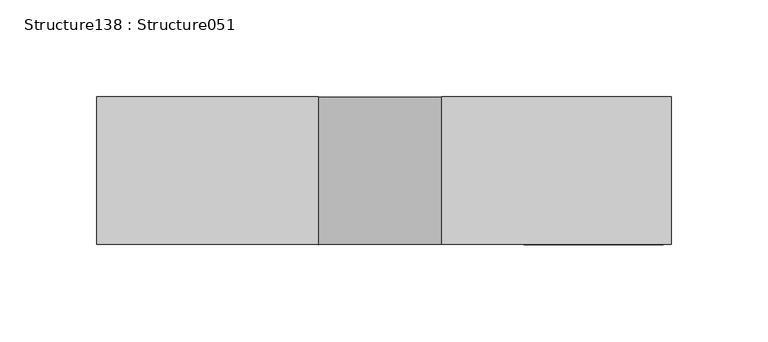
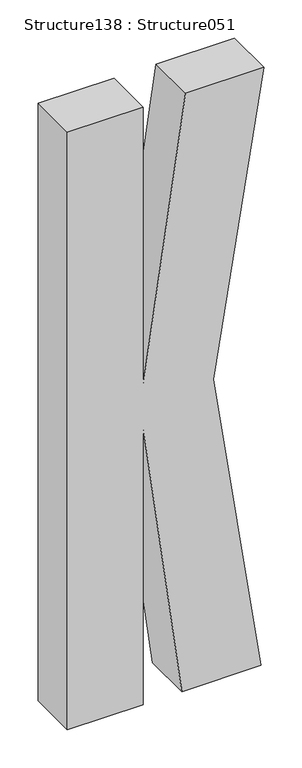
"""IFC4 building model written with IfcOpenShell, lengths in millimetres: proxy geometry, Structure138 : Structure051."""

import ifcopenshell
import ifcopenshell.guid

model = None  # the IFC model being written
_history = None  # IfcOwnerHistory: only IFC2X3 demands one
_inside = {}  # id of a spatial element -> (the spatial element, [elements in it])
_under = {}  # id of a project, library or spatial element -> (it, [spatial elements below it])
_declared = {}  # id of a project -> (the project, [libraries it declares])
_typed = {}  # id of a type object -> (the type object, [elements of that type])
_made_of = {}  # id of a material, layer set ... -> (it, [elements and type objects made of it])


def new_model(schema):
    """Start an empty IFC model of exactly this schema.

    Asked for "IFC4X3", IfcOpenShell would pick the latest addendum, in which some entities
    have other attributes; the version numbers below select the first issue.
    IFC2X3 requires an IfcOwnerHistory on every rooted entity: one is made here for all.
    """
    global model, _history
    if schema == "IFC4X3":
        model = ifcopenshell.file(schema_version=(4, 3, 0, 0))
    else:
        model = ifcopenshell.file(schema=schema)
    _inside.clear()
    _under.clear()
    _declared.clear()
    _typed.clear()
    _made_of.clear()
    _history = None
    if model.schema == "IFC2X3":
        org = make("IfcOrganization", Name="unknown")
        user = make(
            "IfcPersonAndOrganization",
            ThePerson=make("IfcPerson", FamilyName="unknown"),
            TheOrganization=org,
        )
        app = make(
            "IfcApplication",
            ApplicationDeveloper=org,
            Version="unknown",
            ApplicationFullName="unknown",
            ApplicationIdentifier="unknown",
        )
        _history = make(
            "IfcOwnerHistory",
            OwningUser=user,
            OwningApplication=app,
            ChangeAction="ADDED",
            CreationDate=0,
        )
    return model


def make(cls, **values):
    """One entity of the class cls with the attributes given. An attribute that is None is left unset."""
    return model.create_entity(
        cls, **{name: value for name, value in values.items() if value is not None}
    )


def rooted(cls, **values):
    """An entity with a GlobalId (a new one), such as an element, a storey or a relation."""
    return make(cls, GlobalId=ifcopenshell.guid.new(), OwnerHistory=_history, **values)


def si_unit(unit_type, name, prefix=None):
    """IfcSIUnit, for example si_unit("LENGTHUNIT", "METRE", prefix="MILLI")."""
    return make("IfcSIUnit", UnitType=unit_type, Prefix=prefix, Name=name)


def assignment(units):
    """IfcUnitAssignment: the units of a project."""
    return None if units is None else make("IfcUnitAssignment", Units=units)


def point(xyz):
    """IfcCartesianPoint."""
    return None if xyz is None else make("IfcCartesianPoint", Coordinates=xyz)


def direction(xyz):
    """IfcDirection."""
    return None if xyz is None else make("IfcDirection", DirectionRatios=xyz)


def frame(location, z_axis=None, x_axis=None):
    """IfcAxis2Placement3D, a coordinate frame: its origin and axes. An axis left out is left unset."""
    return make(
        "IfcAxis2Placement3D",
        Location=point(location),
        Axis=direction(z_axis),
        RefDirection=direction(x_axis),
    )


def origin():
    """The frame at (0, 0, 0) with its axes left unset."""
    return frame((0.0, 0.0, 0.0))


def place(relative_to, where):
    """IfcLocalPlacement: puts the frame where relative to a parent placement (None: the world)."""
    return make(
        "IfcLocalPlacement", PlacementRelTo=relative_to, RelativePlacement=where
    )


def context(
    kind, dimensions, precision=None, world=None, true_north=None, identifier=None
):
    """IfcGeometricRepresentationContext, for example the 3D "Model" context."""
    return make(
        "IfcGeometricRepresentationContext",
        ContextIdentifier=identifier,
        ContextType=kind,
        CoordinateSpaceDimension=dimensions,
        Precision=precision,
        WorldCoordinateSystem=world,
        TrueNorth=true_north,
    )


def project(units=None, contexts=None):
    """IfcProject with its units and contexts."""
    return rooted(
        "IfcProject",
        Name="project",
        RepresentationContexts=contexts,
        UnitsInContext=assignment(units),
    )


def spatial(cls, under=None, at=None, **own):
    """A site, building, storey or space (cls), placed at a placement, below another one or the project."""
    s = rooted(cls, ObjectPlacement=at, **own)
    if under is not None:
        _under.setdefault(under.id(), (under, []))[1].append(s)
    return s


def polyline(points):
    """IfcPolyline through the points."""
    return make("IfcPolyline", Points=[point(p) for p in points])


def outline(outer, holes=None, kind="AREA"):
    """IfcArbitraryClosedProfileDef: a profile drawn as a closed curve; with holes, ...WithVoids."""
    if holes is None:
        return make("IfcArbitraryClosedProfileDef", ProfileType=kind, OuterCurve=outer)
    return make(
        "IfcArbitraryProfileDefWithVoids",
        ProfileType=kind,
        OuterCurve=outer,
        InnerCurves=holes,
    )


def extrude(swept, where, along, depth):
    """IfcExtrudedAreaSolid: the profile swept, set in the frame where, extruded along a direction by depth."""
    return make(
        "IfcExtrudedAreaSolid",
        SweptArea=swept,
        Position=where,
        ExtrudedDirection=direction(along),
        Depth=depth,
    )


def shape(context_of_items, identifier, shape_type, items):
    """IfcShapeRepresentation: the items that make up one representation, for example the "Body"."""
    return make(
        "IfcShapeRepresentation",
        ContextOfItems=context_of_items,
        RepresentationIdentifier=identifier,
        RepresentationType=shape_type,
        Items=items,
    )


def source(mapping_origin, context_of_items, identifier, shape_type, items):
    """IfcRepresentationMap: a shape defined once, which mapped items show again and again."""
    return make(
        "IfcRepresentationMap",
        MappingOrigin=mapping_origin,
        MappedRepresentation=shape(context_of_items, identifier, shape_type, items),
    )


def transform(
    local_origin,
    x_axis=None,
    y_axis=None,
    z_axis=None,
    scale=None,
    scale2=None,
    scale3=None,
    uniform=True,
):
    """IfcCartesianTransformationOperator3D, or its non-uniform kind. x_axis, y_axis, z_axis: its Axis1, 2, 3."""
    if uniform:
        return make(
            "IfcCartesianTransformationOperator3D",
            Axis1=direction(x_axis),
            Axis2=direction(y_axis),
            LocalOrigin=point(local_origin),
            Scale=scale,
            Axis3=direction(z_axis),
        )
    return make(
        "IfcCartesianTransformationOperator3DnonUniform",
        Axis1=direction(x_axis),
        Axis2=direction(y_axis),
        LocalOrigin=point(local_origin),
        Scale=scale,
        Axis3=direction(z_axis),
        Scale2=scale2,
        Scale3=scale3,
    )


def mapped(mapping_source, mapping_target):
    """IfcMappedItem: shows the shape of a source again, moved by a transform."""
    return make(
        "IfcMappedItem", MappingSource=mapping_source, MappingTarget=mapping_target
    )


def made_of(thing, what):
    """Note that an element or type object is made of a material, layer set ...; save() writes the relation."""
    if what is not None:
        _made_of.setdefault(what.id(), (what, []))[1].append(thing)
    return thing


def element(
    cls,
    number,
    at=None,
    inside=None,
    cuts=None,
    type_object=None,
    material=None,
    context=None,
    identifier="Body",
    shape_type=None,
    held_by="IfcProductDefinitionShape",
    body=None,
    shapes=None,
    **own,
):
    """One element of the class cls, such as IfcWall. Its Tag is "e" and its number.

    at: its placement. inside: the storey or other place that contains it. cuts: it is an
    opening in that element (IfcRelVoidsElement). A single representation is given by context,
    identifier, shape_type and body (its items); several are given by shapes. held_by: the class
    of the entity that holds the representations. save() writes the other relations.
    """
    e = rooted(cls, Tag="e%d" % number, ObjectPlacement=at, **own)
    if body is not None:
        shapes = [shape(context, identifier, shape_type, body)]
    if shapes is not None:
        e.Representation = make(held_by, Representations=shapes)
    if inside is not None:
        _inside.setdefault(inside.id(), (inside, []))[1].append(e)
    if cuts is not None:
        rooted(
            "IfcRelVoidsElement", RelatingBuildingElement=cuts, RelatedOpeningElement=e
        )
    if type_object is not None:
        _typed.setdefault(type_object.id(), (type_object, []))[1].append(e)
    return made_of(e, material)


def aggregate(whole, parts):
    """IfcRelAggregates: a whole, such as a stair, and the parts it consists of."""
    return rooted("IfcRelAggregates", RelatingObject=whole, RelatedObjects=parts)


def save(model, path):
    """Write the relations noted so far, then the file.

    IfcRelAggregates (storeys below a building ...), IfcRelContainedInSpatialStructure (elements
    in a storey), IfcRelDefinesByType, IfcRelAssociatesMaterial and IfcRelDeclares: one each for
    every whole, place, type object, material and project.
    """
    for whole, parts in _under.values():
        aggregate(whole, parts)
    for where, things in _inside.values():
        rooted(
            "IfcRelContainedInSpatialStructure",
            RelatedElements=things,
            RelatingStructure=where,
        )
    for kind, things in _typed.values():
        rooted("IfcRelDefinesByType", RelatedObjects=things, RelatingType=kind)
    for what, things in _made_of.values():
        rooted("IfcRelAssociatesMaterial", RelatedObjects=things, RelatingMaterial=what)
    for by, libraries in _declared.values():
        rooted("IfcRelDeclares", RelatingContext=by, RelatedDefinitions=libraries)
    model.write(path)


def structure138_structure051_ad50acc2(model_context):
    return source(origin(), model_context, "Body", "SweptSolid", [
        extrude(outline(polyline([(3528.5825142, -48176.4103042), (4009.9589531, -48248.4860896), (4480.4419946, -48172.3255164), (4480.4419946, -48290.6288067), (4038.5077532, -48354.5350164), (4480.4419946, -48354.5350164), (4480.4419946, -48468.77934), (3528.5825142, -48468.77934), (3528.5825142, -48354.5350164), (3969.1658661, -48354.5350164), (3528.5825142, -48296.0695224), (3528.5825142, -48176.4103042)])), frame((0.0, 247945.1599557, 0.0), z_axis=(0.0, 1.0, 0.0), x_axis=(0.0, 0.0, 1.0)), (0.0, 0.0, 1.0), 76.2),
    ])


if __name__ == "__main__":
    model = new_model("IFC4")
    model_context = context("Model", 3, world=origin())
    ifc_project = project(units=[si_unit("LENGTHUNIT", "METRE", prefix="MILLI")], contexts=[model_context])
    site = spatial("IfcSite", under=ifc_project)
    building = spatial("IfcBuilding", under=site)
    placement = place(None, origin())
    structure138_structure051_shape = structure138_structure051_ad50acc2(model_context)
    element("IfcBuildingElementProxy", 1, Name="Structure138 : Structure051", ObjectType="Structure138 : Structure051", at=placement, inside=building, context=model_context, shape_type="MappedRepresentation", body=[
        mapped(structure138_structure051_shape, transform((0.0, 0.0, 0.0), x_axis=(1.0, 0.0, 0.0), y_axis=(0.0, 1.0, 0.0), z_axis=(0.0, 0.0, 1.0))),
    ])
    save(model, "model.ifc")

# Revit data of these elements
# Type "Structure138 : Structure051"
#   NameOverride = "Structure051"
# Element 1 (IfcBuildingElementProxy, "Structure138 : Structure051")
#   Materials on its faces: "BRUSHED ALUM. LETTERING"
# Materials
#   "BRUSHED ALUM. LETTERING": class "Unassigned", colour RGB 169 181 186, transparency 0, Cost = 0
